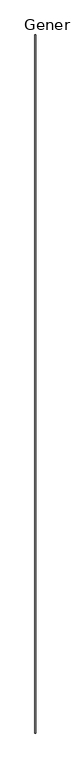
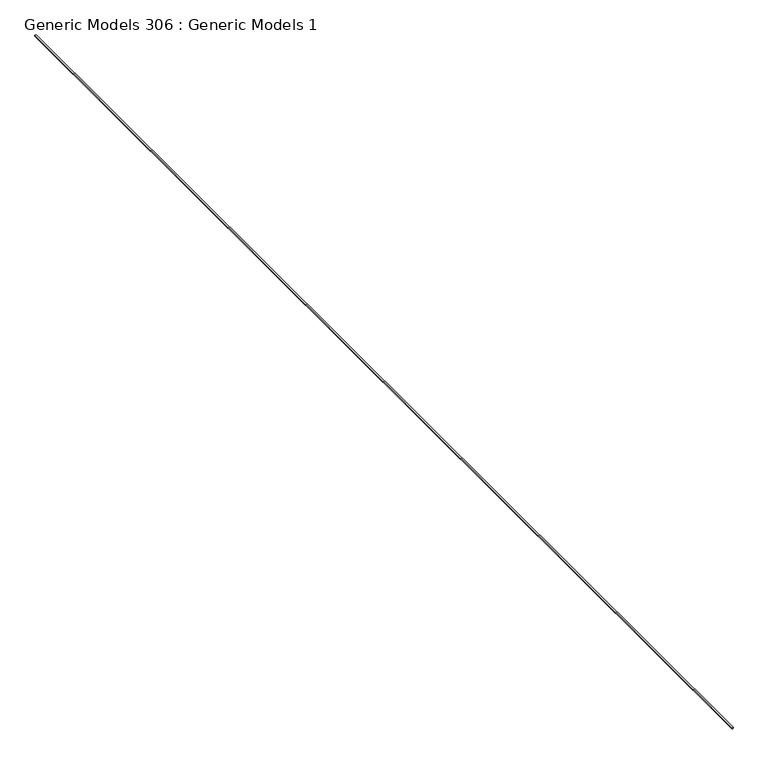
"""IFC4 building model written with IfcOpenShell, lengths in millimetres: proxy geometry, Generic Models 306 : Generic Models 1."""

from ifc_helpers import new_model, si_unit, point, frame, frame_2d, origin, place, context, project, spatial, polyline, circle_curve, trimmed, segment, composite_curve, outline, extrude, source, transform, mapped, element, save


def generic_models_306_generic_models_1_5b98c7ab(model_context):
    return source(origin(), model_context, "Body", "SweptSolid", [
        extrude(outline(composite_curve([segment(polyline([(123145.296, -6924.7940869), (123135.771, -6924.7940869)]), True, "CONTINUOUS"), segment(trimmed(circle_curve(frame_2d((123141.600481, -6918.4440869)), 8.620055), [point((123135.771, -6924.7940869))], [point((123135.771, -6912.0940869))], False, "CARTESIAN"), True, "CONTINUOUS"), segment(polyline([(123135.771, -6912.0940869), (123145.296, -6912.0940869)]), True, "CONTINUOUS"), segment(trimmed(circle_curve(frame_2d((123151.125481, -6918.4440869)), 8.620055), [point((123145.296, -6912.0940869))], [point((123145.296, -6924.7940869))], True, "CARTESIAN"), True, "CONTINUOUS")], self_intersect=False)), frame((0.0, -5493.3230338, 0.0), z_axis=(0.0, 1.0, 0.0), x_axis=(0.0, 0.0, 1.0)), (0.0, 0.0, 1.0), 12344.4),
    ])


if __name__ == "__main__":
    model = new_model("IFC4")
    model_context = context("Model", 3, world=origin())
    ifc_project = project(units=[si_unit("LENGTHUNIT", "METRE", prefix="MILLI")], contexts=[model_context])
    site = spatial("IfcSite", under=ifc_project)
    building = spatial("IfcBuilding", under=site)
    placement = place(None, origin())
    generic_models_306_generic_models_1_shape = generic_models_306_generic_models_1_5b98c7ab(model_context)
    element("IfcBuildingElementProxy", 1, Name="Generic Models 306 : Generic Models 1", ObjectType="Generic Models 306 : Generic Models 1", at=placement, inside=building, context=model_context, shape_type="MappedRepresentation", body=[
        mapped(generic_models_306_generic_models_1_shape, transform((0.0, 0.0, 0.0), x_axis=(1.0, 0.0, 0.0), y_axis=(0.0, 1.0, 0.0), z_axis=(0.0, 0.0, 1.0))),
    ])
    save(model, "model.ifc")

# Revit data of these elements
# Element 1 (IfcBuildingElementProxy, "Generic Models 306 : Generic Models 1")
#   Materials on its faces: "_SEALANT JOINT"
# Materials
#   "_SEALANT JOINT": class "Generic", colour RGB 190 220 196, transparency 0, Cost = 0
